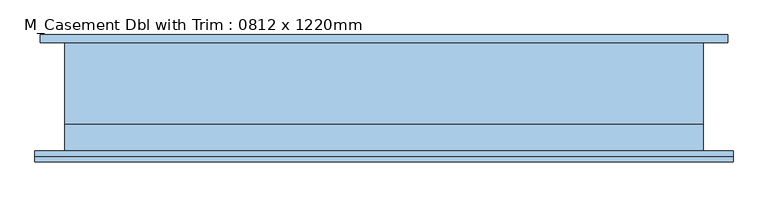
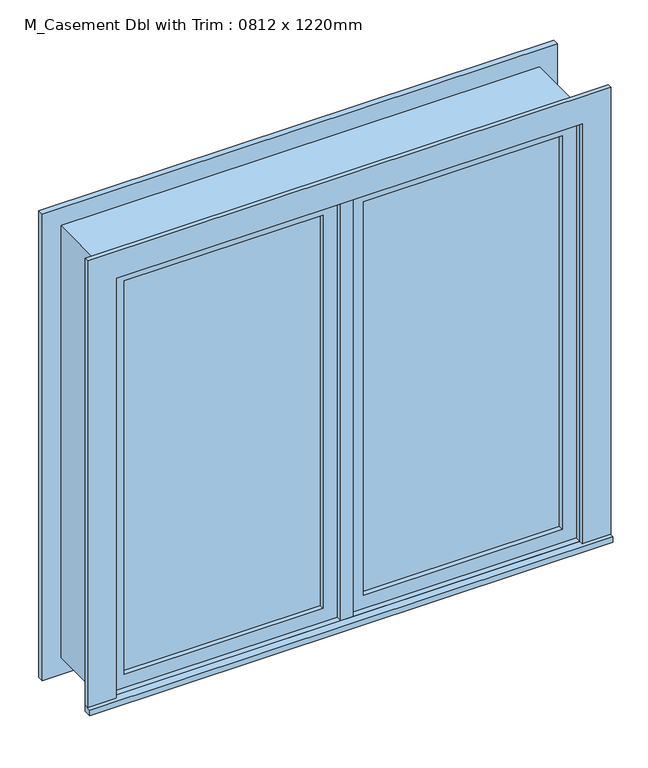
"""IFC4 building model written with IfcOpenShell, lengths in millimetres: window geometry, M_Casement Dbl with Trim : 0812 x 1220mm."""

from ifc_helpers import new_model, si_unit, frame, origin, place, context, project, spatial, polyline, outline, extrude, source, transform, mapped, element, save


def m_casement_dbl_with_trim_0812_x_1220mm_d210905e(model_context):
    return source(origin(), model_context, "Body", "SweptSolid", [
        extrude(outline(polyline([(63.5, -111.175), (63.5, -98.475), (686.5, -98.475), (686.5, -111.175), (63.5, -111.175)])), frame((0.0, 0.0, 963.5), z_axis=(0.0, 0.0, 1.0), x_axis=(1.0, 0.0, 0.0)), (0.0, 0.0, 1.0), 1303.0),
        extrude(outline(polyline([(2310.95, 19.05), (919.05, 19.05), (919.05, 730.95), (2310.95, 730.95), (2310.95, 19.05)]), holes=[polyline([(2266.5, 63.5), (2266.5, 686.5), (963.5, 686.5), (963.5, 63.5), (2266.5, 63.5)])]), frame((0.0, -127.05, 0.0), z_axis=(0.0, 1.0, 0.0), x_axis=(0.0, 0.0, 1.0)), (0.0, 0.0, 1.0), 44.45),
        extrude(outline(polyline([(-819.95, -171.75), (-819.95, -146.05), (819.95, -146.05), (819.95, -171.75), (-819.95, -171.75)])), frame((0.0, 0.0, 900.0), z_axis=(0.0, 0.0, 1.0), x_axis=(1.0, 0.0, 0.0)), (0.0, 0.0, 1.0), 19.05),
        extrude(outline(polyline([(2310.95, -730.95), (2310.95, 730.95), (919.05, 730.95), (919.05, 819.95), (2399.95, 819.95), (2399.95, -819.95), (919.05, -819.95), (919.05, -730.95), (2310.95, -730.95)])), frame((0.0, -159.05, 0.0), z_axis=(0.0, 1.0, 0.0), x_axis=(0.0, 0.0, 1.0)), (0.0, 0.0, 1.0), 13.0),
        extrude(outline(polyline([(2387.25, 807.25), (2387.25, -807.25), (842.75, -807.25), (842.75, 807.25), (2387.25, 807.25)]), holes=[polyline([(2298.25, 718.25), (931.75, 718.25), (931.75, -718.25), (2298.25, -718.25), (2298.25, 718.25)])]), frame((0.0, 107.95, 0.0), z_axis=(0.0, 1.0, 0.0), x_axis=(0.0, 0.0, 1.0)), (0.0, 0.0, 1.0), 19.0),
        extrude(outline(polyline([(-63.5, -98.475), (-63.5, -111.175), (-686.5, -111.175), (-686.5, -98.475), (-63.5, -98.475)])), frame((0.0, 0.0, 963.5), z_axis=(0.0, 0.0, 1.0), x_axis=(1.0, 0.0, 0.0)), (0.0, 0.0, 1.0), 1303.0),
        extrude(outline(polyline([(2310.95, -730.95), (919.05, -730.95), (919.05, -19.05), (2310.95, -19.05), (2310.95, -730.95)]), holes=[polyline([(2266.5, -686.5), (2266.5, -63.5), (963.5, -63.5), (963.5, -686.5), (2266.5, -686.5)])]), frame((0.0, -127.05, 0.0), z_axis=(0.0, 1.0, 0.0), x_axis=(0.0, 0.0, 1.0)), (0.0, 0.0, 1.0), 44.45),
        extrude(outline(polyline([(2330.0, -750.0), (900.0, -750.0), (900.0, 750.0), (2330.0, 750.0), (2330.0, -750.0)]), holes=[polyline([(2298.25, -718.25), (2298.25, 718.25), (931.75, 718.25), (931.75, -718.25), (2298.25, -718.25)])]), frame((0.0, -82.6, 0.0), z_axis=(0.0, 1.0, 0.0), x_axis=(0.0, 0.0, 1.0)), (0.0, 0.0, 1.0), 190.55),
        extrude(outline(polyline([(2330.0, 750.0), (2330.0, -750.0), (900.0, -750.0), (900.0, 750.0), (2330.0, 750.0)]), holes=[polyline([(2310.95, 730.95), (919.05, 730.95), (919.05, -730.95), (2310.95, -730.95), (2310.95, 730.95)])]), frame((0.0, -146.05, 0.0), z_axis=(0.0, 1.0, 0.0), x_axis=(0.0, 0.0, 1.0)), (0.0, 0.0, 1.0), 63.45),
        extrude(outline(polyline([(19.05, -82.6), (19.05, -146.1), (-19.05, -146.1), (-19.05, -82.6), (19.05, -82.6)])), frame((0.0, 0.0, 919.05), z_axis=(0.0, 0.0, 1.0), x_axis=(1.0, 0.0, 0.0)), (0.0, 0.0, 1.0), 1391.9),
    ])


if __name__ == "__main__":
    model = new_model("IFC4")
    model_context = context("Model", 3, world=origin())
    ifc_project = project(units=[si_unit("LENGTHUNIT", "METRE", prefix="MILLI")], contexts=[model_context])
    site = spatial("IfcSite", under=ifc_project)
    building = spatial("IfcBuilding", under=site)
    placement = place(None, origin())
    m_casement_dbl_with_trim_0812_x_1220mm_shape = m_casement_dbl_with_trim_0812_x_1220mm_d210905e(model_context)
    element("IfcWindow", 1, ObjectType="M_Casement Dbl with Trim : 0812 x 1220mm", at=placement, inside=building, context=model_context, shape_type="MappedRepresentation", body=[
        mapped(m_casement_dbl_with_trim_0812_x_1220mm_shape, transform((0.0, 0.0, 0.0), x_axis=(1.0, 0.0, 0.0), y_axis=(0.0, 1.0, 0.0), z_axis=(0.0, 0.0, 1.0))),
    ])
    save(model, "model.ifc")

# Revit data of these elements
# Type "M_Casement Dbl with Trim : 0812 x 1220mm"
#   Type Mark = "W1"
#   Construction Type Id = "GSP4R"
#   Analytic Construction = "1/8 in Pilkington single glazing"
#   Visual Light Transmittance = 0.9
#   Solar Heat Gain Coefficient = 0.78
#   Heat Transfer Coefficient (U) = 3.6886 W/(m²·K)
#   Height = 1430 mm
#   Default Sill Height = 900 mm
#   Trim Projection - Ext. = 13 mm
#   Trim Projection - Int. = 19 mm
#   Trim Width - Exterior = 89 mm
#   Trim Width - Interior = 89 mm
#   Width = 1500 mm
#   Window Inset = 19 mm
#   Glass Pane Material = Glass
#   Sash = wooden-3
#   Trim Exterior Material = wooden-3
#   Trim Interior Material = wooden-3
#   Wall Closure = (empty or 0)
# Element 1 (IfcWindow, "M_Casement Dbl with Trim : 0812 x 1220mm")
#   Materials on its faces: "wooden-3", "Glass"
# Materials
#   "Glass": class "Glass", colour RGB 140 218 255, transparency 0.75, Description = "Soda Lime Glass", Cost = 0
#   "wooden-3": class "Generic", colour RGB 120 120 120, transparency 0, Cost = 0
